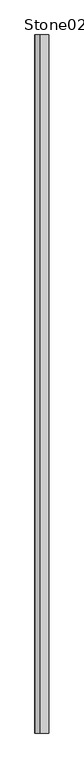
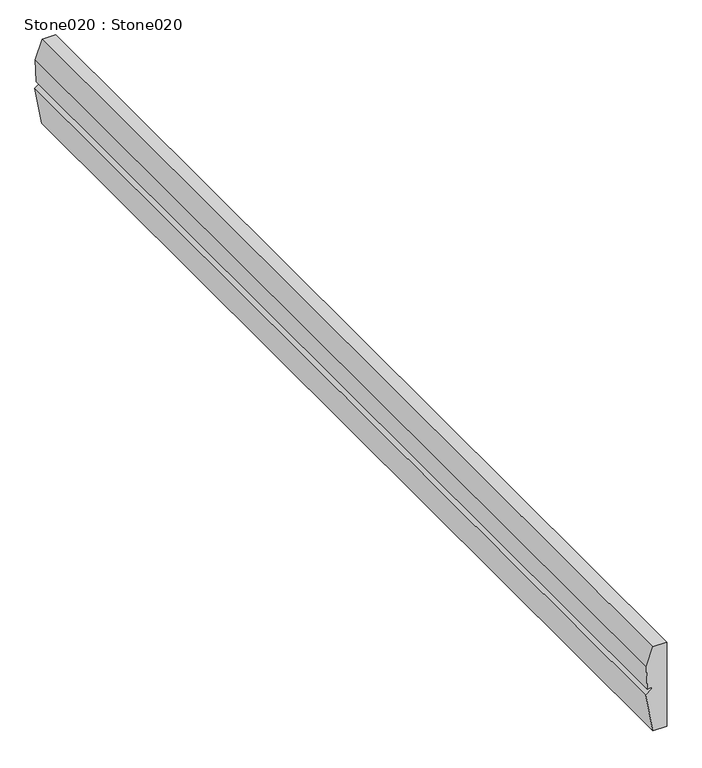
"""IFC4 building model written with IfcOpenShell, lengths in millimetres: proxy geometry, Stone020 : Stone020."""

import ifcopenshell
import ifcopenshell.guid

model = None  # the IFC model being written
_history = None  # IfcOwnerHistory: only IFC2X3 demands one
_inside = {}  # id of a spatial element -> (the spatial element, [elements in it])
_under = {}  # id of a project, library or spatial element -> (it, [spatial elements below it])
_declared = {}  # id of a project -> (the project, [libraries it declares])
_typed = {}  # id of a type object -> (the type object, [elements of that type])
_made_of = {}  # id of a material, layer set ... -> (it, [elements and type objects made of it])


def new_model(schema):
    """Start an empty IFC model of exactly this schema.

    Asked for "IFC4X3", IfcOpenShell would pick the latest addendum, in which some entities
    have other attributes; the version numbers below select the first issue.
    IFC2X3 requires an IfcOwnerHistory on every rooted entity: one is made here for all.
    """
    global model, _history
    if schema == "IFC4X3":
        model = ifcopenshell.file(schema_version=(4, 3, 0, 0))
    else:
        model = ifcopenshell.file(schema=schema)
    _inside.clear()
    _under.clear()
    _declared.clear()
    _typed.clear()
    _made_of.clear()
    _history = None
    if model.schema == "IFC2X3":
        org = make("IfcOrganization", Name="unknown")
        user = make(
            "IfcPersonAndOrganization",
            ThePerson=make("IfcPerson", FamilyName="unknown"),
            TheOrganization=org,
        )
        app = make(
            "IfcApplication",
            ApplicationDeveloper=org,
            Version="unknown",
            ApplicationFullName="unknown",
            ApplicationIdentifier="unknown",
        )
        _history = make(
            "IfcOwnerHistory",
            OwningUser=user,
            OwningApplication=app,
            ChangeAction="ADDED",
            CreationDate=0,
        )
    return model


def make(cls, **values):
    """One entity of the class cls with the attributes given. An attribute that is None is left unset."""
    return model.create_entity(
        cls, **{name: value for name, value in values.items() if value is not None}
    )


def rooted(cls, **values):
    """An entity with a GlobalId (a new one), such as an element, a storey or a relation."""
    return make(cls, GlobalId=ifcopenshell.guid.new(), OwnerHistory=_history, **values)


def si_unit(unit_type, name, prefix=None):
    """IfcSIUnit, for example si_unit("LENGTHUNIT", "METRE", prefix="MILLI")."""
    return make("IfcSIUnit", UnitType=unit_type, Prefix=prefix, Name=name)


def assignment(units):
    """IfcUnitAssignment: the units of a project."""
    return None if units is None else make("IfcUnitAssignment", Units=units)


def point(xyz):
    """IfcCartesianPoint."""
    return None if xyz is None else make("IfcCartesianPoint", Coordinates=xyz)


def direction(xyz):
    """IfcDirection."""
    return None if xyz is None else make("IfcDirection", DirectionRatios=xyz)


def frame(location, z_axis=None, x_axis=None):
    """IfcAxis2Placement3D, a coordinate frame: its origin and axes. An axis left out is left unset."""
    return make(
        "IfcAxis2Placement3D",
        Location=point(location),
        Axis=direction(z_axis),
        RefDirection=direction(x_axis),
    )


def origin():
    """The frame at (0, 0, 0) with its axes left unset."""
    return frame((0.0, 0.0, 0.0))


def place(relative_to, where):
    """IfcLocalPlacement: puts the frame where relative to a parent placement (None: the world)."""
    return make(
        "IfcLocalPlacement", PlacementRelTo=relative_to, RelativePlacement=where
    )


def context(
    kind, dimensions, precision=None, world=None, true_north=None, identifier=None
):
    """IfcGeometricRepresentationContext, for example the 3D "Model" context."""
    return make(
        "IfcGeometricRepresentationContext",
        ContextIdentifier=identifier,
        ContextType=kind,
        CoordinateSpaceDimension=dimensions,
        Precision=precision,
        WorldCoordinateSystem=world,
        TrueNorth=true_north,
    )


def project(units=None, contexts=None):
    """IfcProject with its units and contexts."""
    return rooted(
        "IfcProject",
        Name="project",
        RepresentationContexts=contexts,
        UnitsInContext=assignment(units),
    )


def spatial(cls, under=None, at=None, **own):
    """A site, building, storey or space (cls), placed at a placement, below another one or the project."""
    s = rooted(cls, ObjectPlacement=at, **own)
    if under is not None:
        _under.setdefault(under.id(), (under, []))[1].append(s)
    return s


def polyline(points):
    """IfcPolyline through the points."""
    return make("IfcPolyline", Points=[point(p) for p in points])


def outline(outer, holes=None, kind="AREA"):
    """IfcArbitraryClosedProfileDef: a profile drawn as a closed curve; with holes, ...WithVoids."""
    if holes is None:
        return make("IfcArbitraryClosedProfileDef", ProfileType=kind, OuterCurve=outer)
    return make(
        "IfcArbitraryProfileDefWithVoids",
        ProfileType=kind,
        OuterCurve=outer,
        InnerCurves=holes,
    )


def extrude(swept, where, along, depth):
    """IfcExtrudedAreaSolid: the profile swept, set in the frame where, extruded along a direction by depth."""
    return make(
        "IfcExtrudedAreaSolid",
        SweptArea=swept,
        Position=where,
        ExtrudedDirection=direction(along),
        Depth=depth,
    )


def shape(context_of_items, identifier, shape_type, items):
    """IfcShapeRepresentation: the items that make up one representation, for example the "Body"."""
    return make(
        "IfcShapeRepresentation",
        ContextOfItems=context_of_items,
        RepresentationIdentifier=identifier,
        RepresentationType=shape_type,
        Items=items,
    )


def source(mapping_origin, context_of_items, identifier, shape_type, items):
    """IfcRepresentationMap: a shape defined once, which mapped items show again and again."""
    return make(
        "IfcRepresentationMap",
        MappingOrigin=mapping_origin,
        MappedRepresentation=shape(context_of_items, identifier, shape_type, items),
    )


def transform(
    local_origin,
    x_axis=None,
    y_axis=None,
    z_axis=None,
    scale=None,
    scale2=None,
    scale3=None,
    uniform=True,
):
    """IfcCartesianTransformationOperator3D, or its non-uniform kind. x_axis, y_axis, z_axis: its Axis1, 2, 3."""
    if uniform:
        return make(
            "IfcCartesianTransformationOperator3D",
            Axis1=direction(x_axis),
            Axis2=direction(y_axis),
            LocalOrigin=point(local_origin),
            Scale=scale,
            Axis3=direction(z_axis),
        )
    return make(
        "IfcCartesianTransformationOperator3DnonUniform",
        Axis1=direction(x_axis),
        Axis2=direction(y_axis),
        LocalOrigin=point(local_origin),
        Scale=scale,
        Axis3=direction(z_axis),
        Scale2=scale2,
        Scale3=scale3,
    )


def mapped(mapping_source, mapping_target):
    """IfcMappedItem: shows the shape of a source again, moved by a transform."""
    return make(
        "IfcMappedItem", MappingSource=mapping_source, MappingTarget=mapping_target
    )


def made_of(thing, what):
    """Note that an element or type object is made of a material, layer set ...; save() writes the relation."""
    if what is not None:
        _made_of.setdefault(what.id(), (what, []))[1].append(thing)
    return thing


def element(
    cls,
    number,
    at=None,
    inside=None,
    cuts=None,
    type_object=None,
    material=None,
    context=None,
    identifier="Body",
    shape_type=None,
    held_by="IfcProductDefinitionShape",
    body=None,
    shapes=None,
    **own,
):
    """One element of the class cls, such as IfcWall. Its Tag is "e" and its number.

    at: its placement. inside: the storey or other place that contains it. cuts: it is an
    opening in that element (IfcRelVoidsElement). A single representation is given by context,
    identifier, shape_type and body (its items); several are given by shapes. held_by: the class
    of the entity that holds the representations. save() writes the other relations.
    """
    e = rooted(cls, Tag="e%d" % number, ObjectPlacement=at, **own)
    if body is not None:
        shapes = [shape(context, identifier, shape_type, body)]
    if shapes is not None:
        e.Representation = make(held_by, Representations=shapes)
    if inside is not None:
        _inside.setdefault(inside.id(), (inside, []))[1].append(e)
    if cuts is not None:
        rooted(
            "IfcRelVoidsElement", RelatingBuildingElement=cuts, RelatedOpeningElement=e
        )
    if type_object is not None:
        _typed.setdefault(type_object.id(), (type_object, []))[1].append(e)
    return made_of(e, material)


def aggregate(whole, parts):
    """IfcRelAggregates: a whole, such as a stair, and the parts it consists of."""
    return rooted("IfcRelAggregates", RelatingObject=whole, RelatedObjects=parts)


def save(model, path):
    """Write the relations noted so far, then the file.

    IfcRelAggregates (storeys below a building ...), IfcRelContainedInSpatialStructure (elements
    in a storey), IfcRelDefinesByType, IfcRelAssociatesMaterial and IfcRelDeclares: one each for
    every whole, place, type object, material and project.
    """
    for whole, parts in _under.values():
        aggregate(whole, parts)
    for where, things in _inside.values():
        rooted(
            "IfcRelContainedInSpatialStructure",
            RelatedElements=things,
            RelatingStructure=where,
        )
    for kind, things in _typed.values():
        rooted("IfcRelDefinesByType", RelatedObjects=things, RelatingType=kind)
    for what, things in _made_of.values():
        rooted("IfcRelAssociatesMaterial", RelatedObjects=things, RelatingMaterial=what)
    for by, libraries in _declared.values():
        rooted("IfcRelDeclares", RelatingContext=by, RelatedDefinitions=libraries)
    model.write(path)


def stone020_stone020_adb5f35a(model_context):
    return source(origin(), model_context, "Body", "SweptSolid", [
        extrude(outline(polyline([(32956.2773438, -10292.2685547), (32920.484375, -10304.7431641), (32875.1640625, -10303.0371094), (32876.1835938, -10294.5625), (32872.7304688, -10294.0849609), (32863.9453125, -10305.7998047), (32788.7148438, -10292.7705078), (32788.7148438, -10266.1494141), (32956.2773438, -10266.1494141), (32956.2773438, -10292.2685547)])), frame((0.0, 7982.1531721, 0.0), z_axis=(0.0, 1.0, 0.0), x_axis=(0.0, 0.0, 1.0)), (0.0, 0.0, 1.0), 2000.0),
    ])


if __name__ == "__main__":
    model = new_model("IFC4")
    model_context = context("Model", 3, world=origin())
    ifc_project = project(units=[si_unit("LENGTHUNIT", "METRE", prefix="MILLI")], contexts=[model_context])
    site = spatial("IfcSite", under=ifc_project)
    building = spatial("IfcBuilding", under=site)
    placement = place(None, origin())
    stone020_stone020_shape = stone020_stone020_adb5f35a(model_context)
    element("IfcBuildingElementProxy", 1, Name="Stone020 : Stone020", ObjectType="Stone020 : Stone020", at=placement, inside=building, context=model_context, shape_type="MappedRepresentation", body=[
        mapped(stone020_stone020_shape, transform((0.0, 0.0, 0.0), x_axis=(1.0, 0.0, 0.0), y_axis=(0.0, 1.0, 0.0), z_axis=(0.0, 0.0, 1.0))),
    ])
    save(model, "model.ifc")

# Revit data of these elements
# Type "Stone020 : Stone020"
#   NameOverride = "Stone020"
# Element 1 (IfcBuildingElementProxy, "Stone020 : Stone020")
#   Materials on its faces: "SPLIT FACE STONE 1032"
# Materials
#   "SPLIT FACE STONE 1032": class "Unassigned", colour RGB 205 195 181, transparency 0
